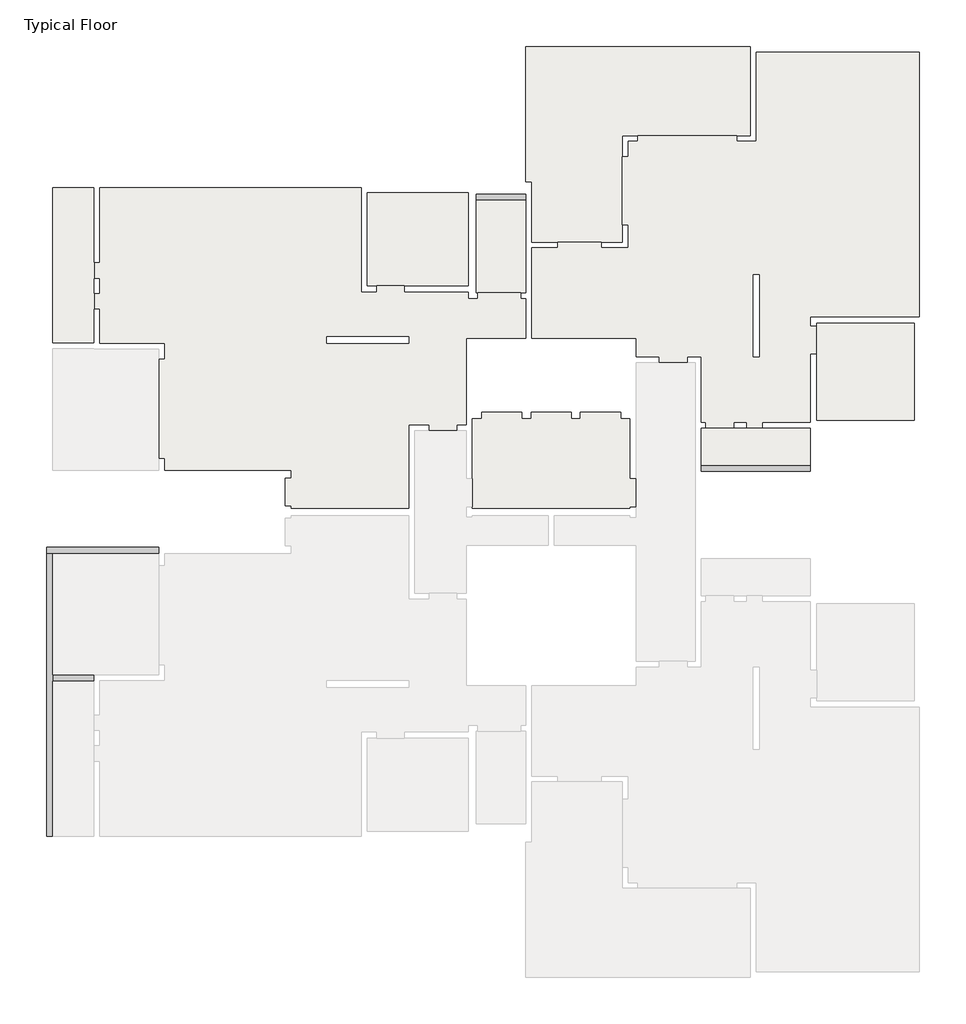
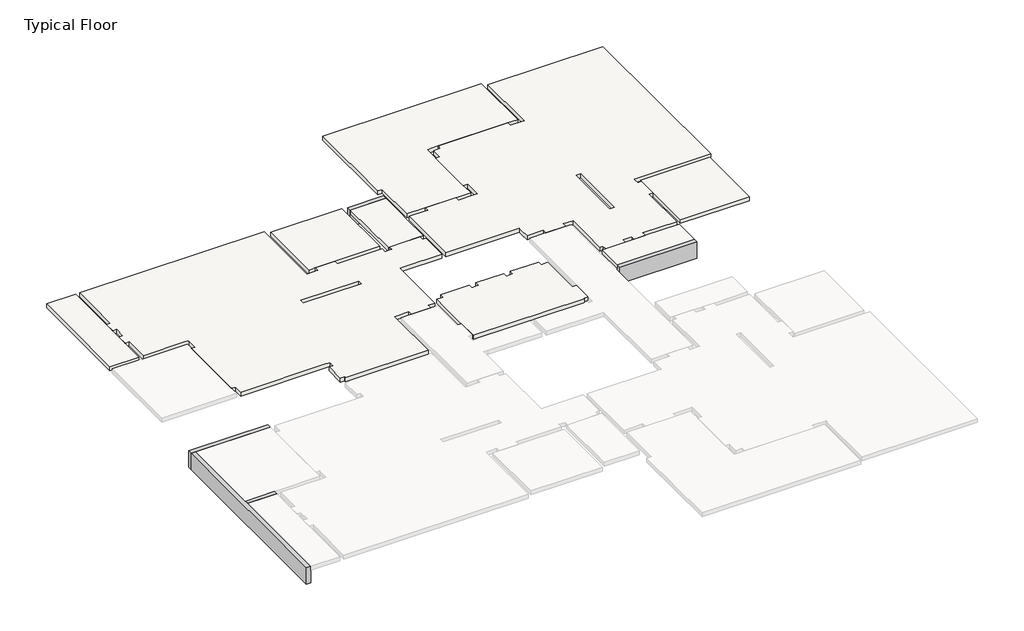
# One storey, part 2 of 2: 9 slabs, 5 beams.
"""IFC4 building model written with IfcOpenShell, lengths in millimetres."""

import ifcopenshell
import ifcopenshell.guid

model = None  # the IFC model being written
_history = None  # IfcOwnerHistory: only IFC2X3 demands one
_inside = {}  # id of a spatial element -> (the spatial element, [elements in it])
_under = {}  # id of a project, library or spatial element -> (it, [spatial elements below it])
_declared = {}  # id of a project -> (the project, [libraries it declares])
_typed = {}  # id of a type object -> (the type object, [elements of that type])
_made_of = {}  # id of a material, layer set ... -> (it, [elements and type objects made of it])


def new_model(schema):
    """Start an empty IFC model of exactly this schema.

    Asked for "IFC4X3", IfcOpenShell would pick the latest addendum, in which some entities
    have other attributes; the version numbers below select the first issue.
    IFC2X3 requires an IfcOwnerHistory on every rooted entity: one is made here for all.
    """
    global model, _history
    if schema == "IFC4X3":
        model = ifcopenshell.file(schema_version=(4, 3, 0, 0))
    else:
        model = ifcopenshell.file(schema=schema)
    _inside.clear()
    _under.clear()
    _declared.clear()
    _typed.clear()
    _made_of.clear()
    _history = None
    if model.schema == "IFC2X3":
        org = make("IfcOrganization", Name="unknown")
        user = make(
            "IfcPersonAndOrganization",
            ThePerson=make("IfcPerson", FamilyName="unknown"),
            TheOrganization=org,
        )
        app = make(
            "IfcApplication",
            ApplicationDeveloper=org,
            Version="unknown",
            ApplicationFullName="unknown",
            ApplicationIdentifier="unknown",
        )
        _history = make(
            "IfcOwnerHistory",
            OwningUser=user,
            OwningApplication=app,
            ChangeAction="ADDED",
            CreationDate=0,
        )
    return model


def make(cls, **values):
    """One entity of the class cls with the attributes given. An attribute that is None is left unset."""
    return model.create_entity(
        cls, **{name: value for name, value in values.items() if value is not None}
    )


def rooted(cls, **values):
    """An entity with a GlobalId (a new one), such as an element, a storey or a relation."""
    return make(cls, GlobalId=ifcopenshell.guid.new(), OwnerHistory=_history, **values)


def si_unit(unit_type, name, prefix=None):
    """IfcSIUnit, for example si_unit("LENGTHUNIT", "METRE", prefix="MILLI")."""
    return make("IfcSIUnit", UnitType=unit_type, Prefix=prefix, Name=name)


def assignment(units):
    """IfcUnitAssignment: the units of a project."""
    return None if units is None else make("IfcUnitAssignment", Units=units)


def point(xyz):
    """IfcCartesianPoint."""
    return None if xyz is None else make("IfcCartesianPoint", Coordinates=xyz)


def direction(xyz):
    """IfcDirection."""
    return None if xyz is None else make("IfcDirection", DirectionRatios=xyz)


def frame(location, z_axis=None, x_axis=None):
    """IfcAxis2Placement3D, a coordinate frame: its origin and axes. An axis left out is left unset."""
    return make(
        "IfcAxis2Placement3D",
        Location=point(location),
        Axis=direction(z_axis),
        RefDirection=direction(x_axis),
    )


def origin():
    """The frame at (0, 0, 0) with its axes left unset."""
    return frame((0.0, 0.0, 0.0))


def place(relative_to, where):
    """IfcLocalPlacement: puts the frame where relative to a parent placement (None: the world)."""
    return make(
        "IfcLocalPlacement", PlacementRelTo=relative_to, RelativePlacement=where
    )


def context(
    kind, dimensions, precision=None, world=None, true_north=None, identifier=None
):
    """IfcGeometricRepresentationContext, for example the 3D "Model" context."""
    return make(
        "IfcGeometricRepresentationContext",
        ContextIdentifier=identifier,
        ContextType=kind,
        CoordinateSpaceDimension=dimensions,
        Precision=precision,
        WorldCoordinateSystem=world,
        TrueNorth=true_north,
    )


def project(units=None, contexts=None):
    """IfcProject with its units and contexts."""
    return rooted(
        "IfcProject",
        Name="project",
        RepresentationContexts=contexts,
        UnitsInContext=assignment(units),
    )


def spatial(cls, under=None, at=None, **own):
    """A site, building, storey or space (cls), placed at a placement, below another one or the project."""
    s = rooted(cls, ObjectPlacement=at, **own)
    if under is not None:
        _under.setdefault(under.id(), (under, []))[1].append(s)
    return s


def faces_of(points, faces, orient=None, outer=None):
    """IfcFace entities. A face is a list of loops; a loop is a list of indices into points, from 0.

    orient and outer hold one flag for each loop. By default every Orientation is true, the
    first loop of a face is its IfcFaceOuterBound and the others are IfcFaceBound.
    """
    made = []
    for i, loops in enumerate(faces):
        bounds = []
        for j, loop in enumerate(loops):
            is_outer = j == 0 if outer is None else outer[i][j]
            bounds.append(
                make(
                    "IfcFaceOuterBound" if is_outer else "IfcFaceBound",
                    Bound=make("IfcPolyLoop", Polygon=[points[k] for k in loop]),
                    Orientation=True if orient is None else orient[i][j],
                )
            )
        made.append(make("IfcFace", Bounds=bounds))
    return made


def faceted_brep(points, faces, orient=None, outer=None, voids=None):
    """IfcFacetedBrep: a solid bounded by flat faces; with voids (closed shells), ...WithVoids."""
    shared = [point(p) for p in points]
    hull = make("IfcClosedShell", CfsFaces=faces_of(shared, faces, orient, outer))
    if voids is None:
        return make("IfcFacetedBrep", Outer=hull)
    return make(
        "IfcFacetedBrepWithVoids",
        Outer=hull,
        Voids=[
            make(cls, CfsFaces=faces_of(shared, fs, o, b)) for cls, fs, o, b in voids
        ],
    )


def shape(context_of_items, identifier, shape_type, items):
    """IfcShapeRepresentation: the items that make up one representation, for example the "Body"."""
    return make(
        "IfcShapeRepresentation",
        ContextOfItems=context_of_items,
        RepresentationIdentifier=identifier,
        RepresentationType=shape_type,
        Items=items,
    )


def made_of(thing, what):
    """Note that an element or type object is made of a material, layer set ...; save() writes the relation."""
    if what is not None:
        _made_of.setdefault(what.id(), (what, []))[1].append(thing)
    return thing


def element(
    cls,
    number,
    at=None,
    inside=None,
    cuts=None,
    type_object=None,
    material=None,
    context=None,
    identifier="Body",
    shape_type=None,
    held_by="IfcProductDefinitionShape",
    body=None,
    shapes=None,
    **own,
):
    """One element of the class cls, such as IfcWall. Its Tag is "e" and its number.

    at: its placement. inside: the storey or other place that contains it. cuts: it is an
    opening in that element (IfcRelVoidsElement). A single representation is given by context,
    identifier, shape_type and body (its items); several are given by shapes. held_by: the class
    of the entity that holds the representations. save() writes the other relations.
    """
    e = rooted(cls, Tag="e%d" % number, ObjectPlacement=at, **own)
    if body is not None:
        shapes = [shape(context, identifier, shape_type, body)]
    if shapes is not None:
        e.Representation = make(held_by, Representations=shapes)
    if inside is not None:
        _inside.setdefault(inside.id(), (inside, []))[1].append(e)
    if cuts is not None:
        rooted(
            "IfcRelVoidsElement", RelatingBuildingElement=cuts, RelatedOpeningElement=e
        )
    if type_object is not None:
        _typed.setdefault(type_object.id(), (type_object, []))[1].append(e)
    return made_of(e, material)


def aggregate(whole, parts):
    """IfcRelAggregates: a whole, such as a stair, and the parts it consists of."""
    return rooted("IfcRelAggregates", RelatingObject=whole, RelatedObjects=parts)


def save(model, path):
    """Write the relations noted so far, then the file.

    IfcRelAggregates (storeys below a building ...), IfcRelContainedInSpatialStructure (elements
    in a storey), IfcRelDefinesByType, IfcRelAssociatesMaterial and IfcRelDeclares: one each for
    every whole, place, type object, material and project.
    """
    for whole, parts in _under.values():
        aggregate(whole, parts)
    for where, things in _inside.values():
        rooted(
            "IfcRelContainedInSpatialStructure",
            RelatedElements=things,
            RelatingStructure=where,
        )
    for kind, things in _typed.values():
        rooted("IfcRelDefinesByType", RelatedObjects=things, RelatingType=kind)
    for what, things in _made_of.values():
        rooted("IfcRelAssociatesMaterial", RelatedObjects=things, RelatingMaterial=what)
    for by, libraries in _declared.values():
        rooted("IfcRelDeclares", RelatingContext=by, RelatedDefinitions=libraries)
    model.write(path)


model = new_model("IFC4")

# Units and contexts
model_context = context("Model", 3, world=origin())
ifc_project = project(units=[si_unit("LENGTHUNIT", "METRE", prefix="MILLI")], contexts=[model_context])

# Site, building, storey
site = spatial("IfcSite", under=ifc_project)
building = spatial("IfcBuilding", under=site)
storey = spatial("IfcBuildingStorey", under=building, Name="Typical Floor", Elevation=3000.0)

# Beams
placement = place(None, origin())
element("IfcBeam", 1, ObjectType="Concrete Rectengular Beam : 20/80", at=placement, inside=storey, context=model_context, shape_type="Brep", body=[
    faceted_brep([(7776.7577342, 13435.0363012, 3000.0), (7776.7577342, 13635.0363012, 3000.0), (4344.3623691, 13635.0363012, 3000.0), (4144.3623691, 13635.0363012, 3000.0), (4144.3623691, 13435.0363012, 3000.0), (4344.3623691, 13435.0363012, 3000.0), (7776.7577342, 13435.0363012, 2200.0), (7776.7577342, 13435.0363012, 2810.0), (4144.3623691, 13435.0363012, 2200.0), (4344.3623691, 13435.0363012, 2200.0), (7776.7577342, 13635.0363012, 2200.0), (4144.3623691, 13635.0363012, 2200.0), (4344.3623691, 13635.0363012, 2200.0)], [[[0, 1, 2, 3, 4, 5]], [[6, 7, 0, 5, 4, 8, 9]], [[10, 6, 9, 8, 11, 12]], [[1, 10, 12, 11, 3, 2]], [[1, 0, 7, 6, 10]], [[4, 3, 11, 8]]]),
])
element("IfcBeam", 2, ObjectType="Concrete Rectengular Beam : 20/80", at=placement, inside=storey, context=model_context, shape_type="Brep", body=[
    faceted_brep([(4144.3623691, 4280.8870961, 3000.0), (4344.3623691, 4280.8870961, 3000.0), (4344.3623691, 9308.461034, 3000.0), (4344.3623691, 9503.461034, 3000.0), (4344.3623691, 13435.0363012, 3000.0), (4144.3623691, 13435.0363012, 3000.0), (4344.3623691, 4280.8870961, 2810.0), (4344.3623691, 4280.8870961, 2200.0), (4344.3623691, 9303.461034, 2200.0), (4344.3623691, 9503.461034, 2200.0), (4344.3623691, 13435.0363012, 2200.0), (4344.3623691, 13435.0363012, 2810.0), (4144.3623691, 4280.8870961, 2200.0), (4144.3623691, 13435.0363012, 2200.0)], [[[0, 1, 2, 3, 4, 5]], [[1, 6, 7, 8, 9, 10, 11, 4, 3, 2]], [[7, 12, 13, 10, 9, 8]], [[12, 0, 5, 13]], [[1, 0, 12, 7, 6]], [[5, 4, 11, 10, 13]]]),
])
element("IfcBeam", 3, ObjectType="Concrete Rectengular Beam : 20/80", at=placement, inside=storey, context=model_context, shape_type="Brep", body=[
    faceted_brep([(5676.0285364, 9503.461034, 3000.0), (4344.3623691, 9503.461034, 3000.0), (4344.3623691, 9308.461034, 3000.0), (5676.0285364, 9308.461034, 3000.0), (4344.3623691, 9303.461034, 2200.0), (5676.0285364, 9303.461034, 2200.0), (5676.0285364, 9303.461034, 2810.0), (4344.3623691, 9303.461034, 2810.0), (5676.0285364, 9503.461034, 2200.0), (4344.3623691, 9503.461034, 2200.0), (4344.3623691, 9503.461034, 2810.0), (5676.0285364, 9308.461034, 2810.0), (4344.3623691, 9308.461034, 2810.0)], [[[0, 1, 2, 3]], [[4, 5, 6, 7]], [[8, 5, 4, 9]], [[9, 10, 1, 0, 8]], [[5, 8, 0, 3, 11, 6]], [[9, 4, 7, 12, 2, 1, 10]], [[11, 12, 7, 6]], [[12, 11, 3, 2]]]),
])
element("IfcBeam", 4, ObjectType="Concrete Rectengular Beam : 20/80", at=placement, inside=storey, context=model_context, shape_type="Brep", body=[
    faceted_brep([(28875.6979001, 16096.9481981, 3000.0), (28875.6979001, 16296.9481981, 3000.0), (25344.8278571, 16296.9481981, 3000.0), (25344.8278571, 16096.9481981, 3000.0), (28875.6979001, 16096.9481981, 2200.0), (25344.8278571, 16096.9481981, 2200.0), (28875.6979001, 16296.9481981, 2200.0), (25344.8278571, 16296.9481981, 2200.0), (28875.6979001, 16296.9481981, 2810.0), (25344.8278571, 16296.9481981, 2810.0)], [[[0, 1, 2, 3]], [[4, 0, 3, 5]], [[6, 4, 5, 7]], [[1, 8, 6, 7, 9, 2]], [[1, 0, 4, 6, 8]], [[3, 2, 9, 7, 5]]]),
])
element("IfcBeam", 5, ObjectType="Concrete Rectengular Beam : 20/80", at=placement, inside=storey, context=model_context, shape_type="Brep", body=[
    faceted_brep([(19662.6522503, 24869.2786346, 3000.0), (19662.6522503, 25069.2786346, 3000.0), (18051.1049523, 25069.2786346, 3000.0), (18051.1049523, 24869.2786346, 3000.0), (19662.6522503, 25069.2786346, 2200.0), (18051.1049523, 25069.2786346, 2200.0), (19662.6522503, 24869.2786346, 2200.0), (18051.1049523, 24869.2786346, 2200.0), (19662.6522503, 24869.2786346, 2810.0), (18051.1049523, 24869.2786346, 2810.0)], [[[0, 1, 2, 3]], [[1, 4, 5, 2]], [[4, 6, 7, 5]], [[6, 8, 0, 3, 9, 7]], [[1, 0, 8, 6, 4]], [[3, 2, 5, 7, 9]]]),
])

# Slabs
element("IfcSlab", 6, ObjectType="19", at=placement, inside=storey, context=model_context, shape_type="Brep", body=[
    faceted_brep([(4344.3623691, 20253.0459905, 2810.0), (4344.3623691, 20258.0459905, 2810.0), (4344.3623691, 25280.6199284, 2810.0), (5676.0285364, 25280.6199284, 2810.0), (5676.0285364, 22851.8697843, 2810.0), (5681.0285364, 22851.8697843, 2810.0), (5681.0285364, 22352.6390151, 2810.0), (5676.0285364, 22352.6390151, 2810.0), (5676.0285364, 21853.4082459, 2810.0), (5681.0285364, 21853.4082459, 2810.0), (5681.0285364, 21354.1774766, 2810.0), (5676.0285364, 21354.1774766, 2810.0), (5676.0285364, 20258.0459905, 2810.0), (5676.0285364, 20253.0459905, 2810.0), (4344.3623691, 25280.6199284, 3000.0), (4344.3623691, 20253.0459905, 3000.0), (5676.0285364, 20253.0459905, 3000.0), (5676.0285364, 21354.1774766, 3000.0), (5681.0285364, 21354.1774766, 3000.0), (5681.0285364, 21853.4082459, 3000.0), (5676.0285364, 21853.4082459, 3000.0), (5676.0285364, 22352.6390151, 3000.0), (5681.0285364, 22352.6390151, 3000.0), (5681.0285364, 22851.8697843, 3000.0), (5676.0285364, 22851.8697843, 3000.0), (5676.0285364, 25280.6199284, 3000.0)], [[[0, 1, 2, 3, 4, 5, 6, 7, 8, 9, 10, 11, 12, 13]], [[14, 15, 16, 17, 18, 19, 20, 21, 22, 23, 24, 25]], [[18, 10, 9, 19]], [[5, 23, 22, 6]], [[15, 0, 13, 16]], [[2, 1, 0, 15, 14]], [[2, 14, 25, 3]], [[11, 17, 16, 13, 12]], [[17, 11, 10, 18]], [[24, 4, 3, 25]], [[4, 24, 23, 5]], [[7, 21, 20, 8]], [[8, 20, 19, 9]], [[21, 7, 6, 22]]]),
])
element("IfcSlab", 7, ObjectType="19", at=placement, inside=storey, context=model_context, shape_type="Brep", body=[
    faceted_brep([(5866.0285364, 22851.8697843, 2810.0), (5866.0285364, 25280.6199284, 2810.0), (14329.4188071, 25280.6199284, 2810.0), (14329.4188071, 22100.4193798, 2810.0), (14329.4188071, 21900.4193798, 2810.0), (14830.1280269, 21900.4193798, 2810.0), (14830.1280269, 22100.4193798, 2810.0), (15730.1380159, 22100.4193798, 2810.0), (15730.1380159, 21900.4193798, 2810.0), (17801.1049523, 21900.4193798, 2810.0), (17801.1049523, 21878.6523235, 2810.0), (17801.1049523, 21688.6523235, 2810.0), (18101.9290458, 21688.6523235, 2810.0), (18101.9290458, 21878.6523235, 2810.0), (19501.7092875, 21878.6523235, 2810.0), (19501.7092875, 21688.6523235, 2810.0), (19662.6522503, 21688.6523235, 2810.0), (19662.6522503, 20409.5793039, 2810.0), (17931.3366974, 20409.5793039, 2810.0), (17731.3366974, 20409.5793039, 2810.0), (17731.3366974, 17607.9011498, 2810.0), (17430.6274775, 17607.9011498, 2810.0), (17430.6274775, 17407.9011498, 2810.0), (16530.6174885, 17407.9011498, 2810.0), (16530.6174885, 17607.9011498, 2810.0), (15871.0829765, 17607.9011498, 2810.0), (15871.0829765, 17407.9011498, 2810.0), (15871.0829765, 14905.7535122, 2810.0), (12068.6856136, 14905.7535122, 2810.0), (12068.6856136, 14975.6366408, 2810.0), (11878.6856136, 14975.6366408, 2810.0), (11878.6856136, 15877.7643004, 2810.0), (12068.6856136, 15877.7643004, 2810.0), (12068.6856136, 16126.4707233, 2810.0), (11878.6856136, 16126.4707233, 2810.0), (7966.7577342, 16126.4707233, 2810.0), (7966.7577342, 16527.889163, 2810.0), (7776.7577342, 16527.889163, 2810.0), (7776.7577342, 19727.6893828, 2810.0), (7966.7577342, 19727.6893828, 2810.0), (7966.7577342, 20248.0459905, 2810.0), (7776.7577342, 20248.0459905, 2810.0), (5866.0285364, 20248.0459905, 2810.0), (5866.0285364, 21354.1774766, 2810.0), (5681.0285364, 21354.1774766, 2810.0), (5681.0285364, 21853.4082459, 2810.0), (5866.0285364, 21853.4082459, 2810.0), (5866.0285364, 22352.6390151, 2810.0), (5681.0285364, 22352.6390151, 2810.0), (5681.0285364, 22851.8697843, 2810.0), (15869.904273, 20448.6363411, 2810.0), (13218.5807289, 20448.6363411, 2810.0), (13218.5807289, 20248.6363411, 2810.0), (15869.904273, 20248.6363411, 2810.0), (5866.0285364, 25280.6199284, 3000.0), (5866.0285364, 22851.8697843, 3000.0), (5681.0285364, 22851.8697843, 3000.0), (5681.0285364, 22352.6390151, 3000.0), (5866.0285364, 22352.6390151, 3000.0), (5866.0285364, 21853.4082459, 3000.0), (5681.0285364, 21853.4082459, 3000.0), (5681.0285364, 21354.1774766, 3000.0), (5866.0285364, 21354.1774766, 3000.0), (5866.0285364, 20248.0459905, 3000.0), (7776.7577342, 20248.0459905, 3000.0), (7966.7577342, 20248.0459905, 3000.0), (7966.7577342, 19727.6893828, 3000.0), (7776.7577342, 19727.6893828, 3000.0), (7776.7577342, 16527.889163, 3000.0), (7966.7577342, 16527.889163, 3000.0), (7966.7577342, 16126.4707233, 3000.0), (11878.6856136, 16126.4707233, 3000.0), (12068.6856136, 16126.4707233, 3000.0), (12068.6856136, 15877.7643004, 3000.0), (11878.6856136, 15877.7643004, 3000.0), (11878.6856136, 14975.6366408, 3000.0), (12068.6856136, 14975.6366408, 3000.0), (12068.6856136, 14905.7535122, 3000.0), (15871.0829765, 14905.7535122, 3000.0), (15871.0829765, 17407.9011498, 3000.0), (15871.0829765, 17607.9011498, 3000.0), (16530.6174885, 17607.9011498, 3000.0), (16530.6174885, 17407.9011498, 3000.0), (17430.6274775, 17407.9011498, 3000.0), (17430.6274775, 17607.9011498, 3000.0), (17731.3366974, 17607.9011498, 3000.0), (17731.3366974, 20409.5793039, 3000.0), (17931.3366974, 20409.5793039, 3000.0), (19662.6522503, 20409.5793039, 3000.0), (19662.6522503, 21688.6523235, 3000.0), (19501.7092875, 21688.6523235, 3000.0), (19501.7092875, 21878.6523235, 3000.0), (18101.9290458, 21878.6523235, 3000.0), (18101.9290458, 21688.6523235, 3000.0), (17801.1049523, 21688.6523235, 3000.0), (17801.1049523, 21878.6523235, 3000.0), (17801.1049523, 21900.4193798, 3000.0), (15730.1380159, 21900.4193798, 3000.0), (15730.1380159, 22100.4193798, 3000.0), (14830.1280269, 22100.4193798, 3000.0), (14830.1280269, 21900.4193798, 3000.0), (14329.4188071, 21900.4193798, 3000.0), (14329.4188071, 22100.4193798, 3000.0), (14329.4188071, 25280.6199284, 3000.0), (13218.5807289, 20448.6363411, 3000.0), (15869.904273, 20448.6363411, 3000.0), (15869.904273, 20248.6363411, 3000.0), (13218.5807289, 20248.6363411, 3000.0)], [[[0, 1, 2, 3, 4, 5, 6, 7, 8, 9, 10, 11, 12, 13, 14, 15, 16, 17, 18, 19, 20, 21, 22, 23, 24, 25, 26, 27, 28, 29, 30, 31, 32, 33, 34, 35, 36, 37, 38, 39, 40, 41, 42, 43, 44, 45, 46, 47, 48, 49], [50, 51, 52, 53]], [[54, 55, 56, 57, 58, 59, 60, 61, 62, 63, 64, 65, 66, 67, 68, 69, 70, 71, 72, 73, 74, 75, 76, 77, 78, 79, 80, 81, 82, 83, 84, 85, 86, 87, 88, 89, 90, 91, 92, 93, 94, 95, 96, 97, 98, 99, 100, 101, 102, 103], [104, 105, 106, 107]], [[1, 0, 55, 54]], [[2, 1, 54, 103]], [[2, 103, 102, 101, 4, 3]], [[5, 4, 101, 100]], [[6, 5, 100, 99]], [[7, 6, 99, 98]], [[8, 7, 98, 97]], [[9, 8, 97, 96]], [[9, 96, 95, 94, 11, 10]], [[12, 11, 94, 93]], [[13, 12, 93, 92]], [[14, 13, 92, 91]], [[15, 14, 91, 90]], [[16, 15, 90, 89]], [[17, 16, 89, 88]], [[17, 88, 87, 86, 19, 18]], [[20, 19, 86, 85]], [[21, 20, 85, 84]], [[22, 21, 84, 83]], [[23, 22, 83, 82]], [[24, 23, 82, 81]], [[25, 24, 81, 80]], [[25, 80, 79, 78, 27, 26]], [[28, 27, 78, 77]], [[29, 28, 77, 76]], [[30, 29, 76, 75]], [[31, 30, 75, 74]], [[32, 31, 74, 73]], [[33, 32, 73, 72]], [[33, 72, 71, 70, 35, 34]], [[36, 35, 70, 69]], [[37, 36, 69, 68]], [[38, 37, 68, 67]], [[39, 38, 67, 66]], [[40, 39, 66, 65]], [[40, 65, 64, 63, 42, 41]], [[43, 42, 63, 62]], [[43, 62, 61, 44]], [[59, 46, 45, 60]], [[47, 46, 59, 58]], [[47, 58, 57, 48]], [[55, 0, 49, 56]], [[51, 50, 105, 104]], [[52, 51, 104, 107]], [[53, 52, 107, 106]], [[50, 53, 106, 105]], [[45, 44, 61, 60]], [[49, 48, 57, 56]]]),
])
element("IfcSlab", 8, ObjectType="19", at=placement, inside=storey, context=model_context, shape_type="Brep", body=[
    faceted_brep([(23233.0448184, 20409.5793039, 2810.0), (19852.6522503, 20409.5793039, 2810.0), (19852.6522503, 23329.8470094, 2810.0), (20702.4284964, 23329.8470094, 2810.0), (20702.4284964, 23519.8470094, 2810.0), (22104.3264087, 23519.8470094, 2810.0), (22104.3264087, 23329.8470094, 2810.0), (22784.6890098, 23329.8470094, 2810.0), (22974.6890098, 23329.8470094, 2810.0), (22974.6890098, 24081.620059, 2810.0), (22784.6890098, 24081.620059, 2810.0), (22784.0986592, 24081.620059, 2810.0), (22784.0986592, 26281.8797734, 2810.0), (22974.0986592, 26281.8797734, 2810.0), (22974.0986592, 26781.6500261, 2810.0), (23288.1042531, 26781.6500261, 2810.0), (23288.1042531, 26971.6500261, 2810.0), (26490.0221434, 26971.6500261, 2810.0), (26490.0221434, 26781.6500261, 2810.0), (27124.7329615, 26781.6500261, 2810.0), (27124.7329615, 26971.6500261, 2810.0), (27124.7329615, 29662.2723415, 2810.0), (32407.3840453, 29662.2723415, 2810.0), (32407.3840453, 21099.9399072, 2810.0), (29076.6368672, 21099.9399072, 2810.0), (28876.6368672, 21099.9399072, 2810.0), (28876.6368672, 20799.2306873, 2810.0), (29076.6368672, 20799.2306873, 2810.0), (29076.6368672, 19899.2206983, 2810.0), (28876.6368672, 19899.2206983, 2810.0), (28876.6368672, 17688.3726312, 2810.0), (27326.5020155, 17688.3726312, 2810.0), (27326.5020155, 17488.3726312, 2810.0), (26824.6140922, 17488.3726312, 2810.0), (26824.6140922, 17688.3726312, 2810.0), (26394.7269681, 17688.3726312, 2810.0), (26394.7269681, 17488.3726312, 2810.0), (25494.7169791, 17488.3726312, 2810.0), (25494.7169791, 17688.3726312, 2810.0), (25344.8278571, 17688.3726312, 2810.0), (25344.8278571, 19609.0998313, 2810.0), (25344.8278571, 19809.0998313, 2810.0), (24884.8278571, 19809.0998313, 2810.0), (24884.8278571, 19609.0998313, 2810.0), (23984.8178681, 19609.0998313, 2810.0), (23984.8178681, 19809.0998313, 2810.0), (23233.0448184, 19809.0998313, 2810.0), (23233.0448184, 20209.5793039, 2810.0), (27225.7927957, 19808.1608642, 2810.0), (27225.7927957, 22459.4844083, 2810.0), (27025.7927957, 22459.4844083, 2810.0), (27025.7927957, 19808.1608642, 2810.0), (19852.6522503, 20409.5793039, 3000.0), (23233.0448184, 20409.5793039, 3000.0), (23233.0448184, 20209.5793039, 3000.0), (23233.0448184, 19809.0998313, 3000.0), (23984.8178681, 19809.0998313, 3000.0), (23984.8178681, 19609.0998313, 3000.0), (24884.8278571, 19609.0998313, 3000.0), (24884.8278571, 19809.0998313, 3000.0), (25344.8278571, 19809.0998313, 3000.0), (25344.8278571, 19609.0998313, 3000.0), (25344.8278571, 17688.3726312, 3000.0), (25494.7169791, 17688.3726312, 3000.0), (25494.7169791, 17488.3726312, 3000.0), (26394.7269681, 17488.3726312, 3000.0), (26394.7269681, 17688.3726312, 3000.0), (26824.6140922, 17688.3726312, 3000.0), (26824.6140922, 17488.3726312, 3000.0), (27326.5020155, 17488.3726312, 3000.0), (27326.5020155, 17688.3726312, 3000.0), (28876.6368672, 17688.3726312, 3000.0), (28876.6368672, 19899.2206983, 3000.0), (29076.6368672, 19899.2206983, 3000.0), (29076.6368672, 20799.2306873, 3000.0), (28876.6368672, 20799.2306873, 3000.0), (28876.6368672, 21099.9399072, 3000.0), (29076.6368672, 21099.9399072, 3000.0), (32407.3840453, 21099.9399072, 3000.0), (32407.3840453, 29662.2723415, 3000.0), (27124.7329615, 29662.2723415, 3000.0), (27124.7329615, 26971.6500261, 3000.0), (27124.7329615, 26781.6500261, 3000.0), (26490.0221434, 26781.6500261, 3000.0), (26490.0221434, 26971.6500261, 3000.0), (23288.1042531, 26971.6500261, 3000.0), (23288.1042531, 26781.6500261, 3000.0), (22974.0986592, 26781.6500261, 3000.0), (22974.0986592, 26281.8797734, 3000.0), (22784.0986592, 26281.8797734, 3000.0), (22784.0986592, 24081.620059, 3000.0), (22784.6890098, 24081.620059, 3000.0), (22974.6890098, 24081.620059, 3000.0), (22974.6890098, 23329.8470094, 3000.0), (22784.6890098, 23329.8470094, 3000.0), (22104.3264087, 23329.8470094, 3000.0), (22104.3264087, 23519.8470094, 3000.0), (20702.4284964, 23519.8470094, 3000.0), (20702.4284964, 23329.8470094, 3000.0), (19852.6522503, 23329.8470094, 3000.0), (27225.7927957, 22459.4844083, 3000.0), (27225.7927957, 19808.1608642, 3000.0), (27025.7927957, 19808.1608642, 3000.0), (27025.7927957, 22459.4844083, 3000.0)], [[[0, 1, 2, 3, 4, 5, 6, 7, 8, 9, 10, 11, 12, 13, 14, 15, 16, 17, 18, 19, 20, 21, 22, 23, 24, 25, 26, 27, 28, 29, 30, 31, 32, 33, 34, 35, 36, 37, 38, 39, 40, 41, 42, 43, 44, 45, 46, 47], [48, 49, 50, 51]], [[52, 53, 54, 55, 56, 57, 58, 59, 60, 61, 62, 63, 64, 65, 66, 67, 68, 69, 70, 71, 72, 73, 74, 75, 76, 77, 78, 79, 80, 81, 82, 83, 84, 85, 86, 87, 88, 89, 90, 91, 92, 93, 94, 95, 96, 97, 98, 99], [100, 101, 102, 103]], [[1, 0, 53, 52]], [[2, 1, 52, 99]], [[3, 2, 99, 98]], [[4, 3, 98, 97]], [[5, 4, 97, 96]], [[6, 5, 96, 95]], [[6, 95, 94, 93, 8, 7]], [[9, 8, 93, 92]], [[9, 92, 91, 90, 11, 10]], [[12, 11, 90, 89]], [[13, 12, 89, 88]], [[14, 13, 88, 87]], [[15, 14, 87, 86]], [[16, 15, 86, 85]], [[17, 16, 85, 84]], [[18, 17, 84, 83]], [[19, 18, 83, 82]], [[19, 82, 81, 80, 21, 20]], [[22, 21, 80, 79]], [[23, 22, 79, 78]], [[23, 78, 77, 76, 25, 24]], [[26, 25, 76, 75]], [[27, 26, 75, 74]], [[28, 27, 74, 73]], [[29, 28, 73, 72]], [[30, 29, 72, 71]], [[31, 30, 71, 70]], [[32, 31, 70, 69]], [[33, 32, 69, 68]], [[34, 33, 68, 67]], [[35, 34, 67, 66]], [[36, 35, 66, 65]], [[37, 36, 65, 64]], [[38, 37, 64, 63]], [[39, 38, 63, 62]], [[39, 62, 61, 60, 41, 40]], [[42, 41, 60, 59]], [[43, 42, 59, 58]], [[44, 43, 58, 57]], [[45, 44, 57, 56]], [[46, 45, 56, 55]], [[46, 55, 54, 53, 0, 47]], [[48, 101, 100, 49]], [[50, 103, 102, 51]], [[49, 100, 103, 50]], [[101, 48, 51, 102]]]),
])
element("IfcSlab", 9, ObjectType="19", at=placement, inside=storey, context=model_context, shape_type="Brep", body=[
    faceted_brep([(29076.6368672, 20899.9399072, 2810.0), (32247.3840453, 20899.9399072, 2810.0), (32247.3840453, 17747.7822806, 2810.0), (29076.6368672, 17747.7822806, 2810.0), (29076.6368672, 19899.2206983, 2810.0), (29076.6368672, 20799.2306873, 2810.0), (32247.3840453, 20899.9399072, 3000.0), (29076.6368672, 20899.9399072, 3000.0), (29076.6368672, 20799.2306873, 3000.0), (29076.6368672, 19899.2206983, 3000.0), (29076.6368672, 17747.7822806, 3000.0), (32247.3840453, 17747.7822806, 3000.0)], [[[0, 1, 2, 3, 4, 5]], [[6, 7, 8, 9, 10, 11]], [[1, 0, 7, 6]], [[2, 1, 6, 11]], [[3, 2, 11, 10]], [[3, 10, 9, 8, 7, 0, 5, 4]]]),
])
element("IfcSlab", 10, ObjectType="19", at=placement, inside=storey, context=model_context, shape_type="Brep", body=[
    faceted_brep([(19662.6522503, 29852.2723415, 2810.0), (26934.7329615, 29852.2723415, 2810.0), (26934.7329615, 26971.6500261, 2810.0), (26490.0221434, 26971.6500261, 2810.0), (23288.1042531, 26971.6500261, 2810.0), (22784.0986592, 26971.6500261, 2810.0), (22784.0986592, 26281.8797734, 2810.0), (22784.0986592, 24081.620059, 2810.0), (22784.6890098, 24081.620059, 2810.0), (22784.6890098, 23519.8470094, 2810.0), (22104.3264087, 23519.8470094, 2810.0), (20702.4284964, 23519.8470094, 2810.0), (19852.6522503, 23519.8470094, 2810.0), (19852.6522503, 25470.811948, 2810.0), (19662.6522503, 25470.811948, 2810.0), (26934.7329615, 29852.2723415, 3000.0), (19662.6522503, 29852.2723415, 3000.0), (19662.6522503, 25470.811948, 3000.0), (19852.6522503, 25470.811948, 3000.0), (19852.6522503, 23519.8470094, 3000.0), (20702.4284964, 23519.8470094, 3000.0), (22104.3264087, 23519.8470094, 3000.0), (22784.6890098, 23519.8470094, 3000.0), (22784.6890098, 24081.620059, 3000.0), (22784.0986592, 24081.620059, 3000.0), (22784.0986592, 26281.8797734, 3000.0), (22784.0986592, 26971.6500261, 3000.0), (22974.0986592, 26971.6500261, 3000.0), (23288.1042531, 26971.6500261, 3000.0), (26490.0221434, 26971.6500261, 3000.0), (26934.7329615, 26971.6500261, 3000.0), (26934.7329615, 29662.2723415, 3000.0)], [[[0, 1, 2, 3, 4, 5, 6, 7, 8, 9, 10, 11, 12, 13, 14]], [[15, 16, 17, 18, 19, 20, 21, 22, 23, 24, 25, 26, 27, 28, 29, 30, 31]], [[1, 0, 16, 15]], [[2, 1, 15, 31, 30]], [[2, 30, 29, 28, 27, 26, 5, 4, 3]], [[19, 12, 11, 10, 9, 22, 21, 20]], [[13, 12, 19, 18]], [[14, 13, 18, 17]], [[0, 14, 17, 16]], [[5, 26, 25, 24, 7, 6]], [[9, 8, 23, 22]], [[7, 24, 23, 8]]]),
])
element("IfcSlab", 11, ObjectType="19", at=placement, inside=storey, context=model_context, shape_type="Brep", body=[
    faceted_brep([(14529.4188071, 22100.4193798, 2810.0), (14529.4188071, 25120.7159382, 2810.0), (17801.1049523, 25120.7159382, 2810.0), (17801.1049523, 22100.4193798, 2810.0), (15730.1380159, 22100.4193798, 2810.0), (14830.1280269, 22100.4193798, 2810.0), (14529.4188071, 25120.7159382, 3000.0), (14529.4188071, 22100.4193798, 3000.0), (14830.1280269, 22100.4193798, 3000.0), (15730.1380159, 22100.4193798, 3000.0), (17801.1049523, 22100.4193798, 3000.0), (17801.1049523, 25120.7159382, 3000.0)], [[[0, 1, 2, 3, 4, 5]], [[6, 7, 8, 9, 10, 11]], [[7, 0, 5, 4, 3, 10, 9, 8]], [[1, 0, 7, 6]], [[2, 1, 6, 11]], [[3, 2, 11, 10]]]),
])
element("IfcSlab", 12, ObjectType="19", at=placement, inside=storey, context=model_context, shape_type="Brep", body=[
    faceted_brep([(17931.3366974, 17808.1408861, 2810.0), (18231.1069501, 17808.1408861, 2810.0), (18231.1069501, 18008.1408861, 2810.0), (19531.3566754, 18008.1408861, 2810.0), (19531.3566754, 17808.1408861, 2810.0), (19832.0658953, 17808.1408861, 2810.0), (19832.0658953, 18008.1408861, 2810.0), (21132.3156206, 18008.1408861, 2810.0), (21132.3156206, 17808.1408861, 2810.0), (21433.0248404, 17808.1408861, 2810.0), (21433.0248404, 18008.1408861, 2810.0), (22733.2745657, 18008.1408861, 2810.0), (22733.2745657, 17808.1408861, 2810.0), (23033.0448184, 17808.1408861, 2810.0), (23033.0448184, 15856.5875947, 2810.0), (23233.0448184, 15856.5875947, 2810.0), (23233.0448184, 14956.5776057, 2810.0), (23033.0448184, 14956.5776057, 2810.0), (23033.0448184, 14905.8683859, 2810.0), (17931.3366974, 14905.8683859, 2810.0), (17931.3366974, 14956.5776057, 2810.0), (17931.3366974, 15852.9011498, 2810.0), (18231.1069501, 17808.1408861, 3000.0), (17931.3366974, 17808.1408861, 3000.0), (17931.3366974, 15852.9011498, 3000.0), (17931.3366974, 14956.5776057, 3000.0), (17931.3366974, 14905.8683859, 3000.0), (23033.0448184, 14905.8683859, 3000.0), (23033.0448184, 14956.5776057, 3000.0), (23233.0448184, 14956.5776057, 3000.0), (23233.0448184, 15856.5875947, 3000.0), (23033.0448184, 15856.5875947, 3000.0), (23033.0448184, 17808.1408861, 3000.0), (22733.2745657, 17808.1408861, 3000.0), (22733.2745657, 18008.1408861, 3000.0), (21433.0248404, 18008.1408861, 3000.0), (21433.0248404, 17808.1408861, 3000.0), (21132.3156206, 17808.1408861, 3000.0), (21132.3156206, 18008.1408861, 3000.0), (19832.0658953, 18008.1408861, 3000.0), (19832.0658953, 17808.1408861, 3000.0), (19531.3566754, 17808.1408861, 3000.0), (19531.3566754, 18008.1408861, 3000.0), (18231.1069501, 18008.1408861, 3000.0)], [[[0, 1, 2, 3, 4, 5, 6, 7, 8, 9, 10, 11, 12, 13, 14, 15, 16, 17, 18, 19, 20, 21]], [[22, 23, 24, 25, 26, 27, 28, 29, 30, 31, 32, 33, 34, 35, 36, 37, 38, 39, 40, 41, 42, 43]], [[1, 0, 23, 22]], [[2, 1, 22, 43]], [[3, 2, 43, 42]], [[4, 3, 42, 41]], [[5, 4, 41, 40]], [[6, 5, 40, 39]], [[7, 6, 39, 38]], [[8, 7, 38, 37]], [[9, 8, 37, 36]], [[10, 9, 36, 35]], [[11, 10, 35, 34]], [[12, 11, 34, 33]], [[13, 12, 33, 32]], [[14, 13, 32, 31]], [[15, 14, 31, 30]], [[16, 15, 30, 29]], [[17, 16, 29, 28]], [[18, 17, 28, 27]], [[19, 18, 27, 26]], [[19, 26, 25, 24, 23, 0, 21, 20]]]),
])
element("IfcSlab", 13, ObjectType="19", at=placement, inside=storey, context=model_context, shape_type="Brep", body=[
    faceted_brep([(19662.6522503, 24869.2786346, 2810.0), (19662.6522503, 21878.6523235, 2810.0), (19501.7092875, 21878.6523235, 2810.0), (18101.9290458, 21878.6523235, 2810.0), (18051.1049523, 21878.6523235, 2810.0), (18051.1049523, 24869.2786346, 2810.0), (19662.6522503, 21878.6523235, 3000.0), (19662.6522503, 23329.8470094, 3000.0), (19662.6522503, 23519.8470094, 3000.0), (19662.6522503, 24869.2786346, 3000.0), (18051.1049523, 24869.2786346, 3000.0), (18051.1049523, 21878.6523235, 3000.0), (18101.9290458, 21878.6523235, 3000.0), (19501.7092875, 21878.6523235, 3000.0)], [[[0, 1, 2, 3, 4, 5]], [[6, 7, 8, 9, 10, 11, 12, 13]], [[1, 0, 9, 8, 7, 6]], [[0, 5, 10, 9]], [[5, 4, 11, 10]], [[11, 4, 3, 2, 1, 6, 13, 12]]]),
])
element("IfcSlab", 14, ObjectType="19", at=placement, inside=storey, context=model_context, shape_type="Brep", body=[
    faceted_brep([(28875.6979001, 16296.9481981, 2810.0), (25344.8278571, 16296.9481981, 2810.0), (25344.8278571, 17488.3726312, 2810.0), (25494.7169791, 17488.3726312, 2810.0), (26394.7269681, 17488.3726312, 2810.0), (26824.6140922, 17488.3726312, 2810.0), (27326.5020155, 17488.3726312, 2810.0), (28875.6979001, 17488.3726312, 2810.0), (28875.6979001, 16296.9481981, 3000.0), (28875.6979001, 17488.3726312, 3000.0), (27326.5020155, 17488.3726312, 3000.0), (26824.6140922, 17488.3726312, 3000.0), (26394.7269681, 17488.3726312, 3000.0), (25494.7169791, 17488.3726312, 3000.0), (25344.8278571, 17488.3726312, 3000.0), (25344.8278571, 16296.9481981, 3000.0)], [[[0, 1, 2, 3, 4, 5, 6, 7]], [[8, 9, 10, 11, 12, 13, 14, 15]], [[0, 7, 9, 8]], [[7, 6, 5, 4, 3, 2, 14, 13, 12, 11, 10, 9]], [[2, 1, 15, 14]], [[1, 0, 8, 15]]]),
])

save(model, "model.ifc")

# Revit data of these elements
# Type "Concrete Rectengular Beam : 20/80"
#   Length [instance default] = 152.4 cm
#   b = 20 cm
#   h = 80 cm
#   Structural Material [instance default] = Concrete
#   Assembly Code = ""
# Type "19"
#   Function = 0
#   Layers, outside or top first: 19 cm "Concrete" (function 1)
# Element 1 (IfcBeam, "Concrete Rectengular Beam : 20/80")
#   Comments = ""
#   Mark = "B4"
#   SOFiSTiK_AMG_Comments = ""
#   SOFiSTiK_AMG_Scheduled = yes
#   SOFiSTiK_AMG_Adjusted = yes
#   Structural Material = Concrete
#   Phase Created = New Construction
#   Materials on its faces: "Concrete"
# Element 2 (IfcBeam, "Concrete Rectengular Beam : 20/80")
#   Comments = ""
#   Mark = "B5"
#   SOFiSTiK_AMG_Comments = ""
#   SOFiSTiK_AMG_Scheduled = yes
#   SOFiSTiK_AMG_Adjusted = yes
#   Structural Material = Concrete
#   Phase Created = New Construction
#   Materials on its faces: "Concrete"
# Element 3 (IfcBeam, "Concrete Rectengular Beam : 20/80")
#   Comments = ""
#   Mark = "B6"
#   SOFiSTiK_AMG_Comments = ""
#   SOFiSTiK_AMG_Scheduled = yes
#   SOFiSTiK_AMG_Adjusted = yes
#   Structural Material = Concrete
#   Phase Created = New Construction
#   Materials on its faces: "Concrete"
# Element 4 (IfcBeam, "Concrete Rectengular Beam : 20/80")
#   Comments = ""
#   Mark = "B10"
#   SOFiSTiK_AMG_Comments = ""
#   SOFiSTiK_AMG_Scheduled = yes
#   SOFiSTiK_AMG_Adjusted = yes
#   Structural Material = Concrete
#   Phase Created = New Construction
#   Materials on its faces: "Concrete"
# Element 5 (IfcBeam, "Concrete Rectengular Beam : 20/80")
#   Comments = ""
#   Mark = "B11"
#   SOFiSTiK_AMG_Comments = ""
#   SOFiSTiK_AMG_Scheduled = yes
#   SOFiSTiK_AMG_Adjusted = yes
#   Structural Material = Concrete
#   Phase Created = New Construction
#   Materials on its faces: "Concrete"
# Element 6 (IfcSlab, "19")
#   Mark = "S2"
#   SOFiSTiK_AMG_Comments = ""
#   Height Offset From Level = 0 cm
#   built-in parameter 1001954 = 1
#   SOFiSTiK_AMG_Scheduled = yes
#   SOFiSTiK_AMG_Adjusted = yes
#   Phase Created = New Construction
#   Materials on its faces: "Concrete"
# Element 7 (IfcSlab, "19")
#   Mark = "S3"
#   SOFiSTiK_AMG_Comments = ""
#   built-in parameter 1001955 = -1.5708 (stored number, unit not read)
#   Height Offset From Level = 0 cm
#   built-in parameter 1001954 = 1
#   SOFiSTiK_AMG_Scheduled = yes
#   SOFiSTiK_AMG_Adjusted = yes
#   Phase Created = New Construction
#   Materials on its faces: "Concrete"
# Element 8 (IfcSlab, "19")
#   Mark = "S4"
#   SOFiSTiK_AMG_Comments = ""
#   Height Offset From Level = 0 cm
#   built-in parameter 1001954 = 1
#   SOFiSTiK_AMG_Scheduled = yes
#   SOFiSTiK_AMG_Adjusted = yes
#   Phase Created = New Construction
#   Materials on its faces: "Concrete"
# Element 9 (IfcSlab, "19")
#   Mark = "S5"
#   SOFiSTiK_AMG_Comments = ""
#   built-in parameter 1001955 = 3.14159 (stored number, unit not read)
#   Height Offset From Level = 0 cm
#   built-in parameter 1001954 = 1
#   SOFiSTiK_AMG_Scheduled = yes
#   SOFiSTiK_AMG_Adjusted = yes
#   Phase Created = New Construction
#   Materials on its faces: "Concrete"
# Element 10 (IfcSlab, "19")
#   Mark = "S6"
#   SOFiSTiK_AMG_Comments = ""
#   built-in parameter 1001955 = 1.5708 (stored number, unit not read)
#   Height Offset From Level = 0 cm
#   built-in parameter 1001954 = 1
#   SOFiSTiK_AMG_Scheduled = yes
#   SOFiSTiK_AMG_Adjusted = yes
#   Phase Created = New Construction
#   Materials on its faces: "Concrete"
# Element 11 (IfcSlab, "19")
#   Mark = "S7"
#   SOFiSTiK_AMG_Comments = ""
#   Height Offset From Level = 0 cm
#   built-in parameter 1001954 = 1
#   SOFiSTiK_AMG_Scheduled = yes
#   SOFiSTiK_AMG_Adjusted = yes
#   Phase Created = New Construction
#   Materials on its faces: "Concrete"
# Element 12 (IfcSlab, "19")
#   Mark = "S17"
#   SOFiSTiK_AMG_Comments = ""
#   built-in parameter 1001955 = 1.5708 (stored number, unit not read)
#   Height Offset From Level = 0 cm
#   built-in parameter 1001954 = 1
#   SOFiSTiK_AMG_Scheduled = yes
#   SOFiSTiK_AMG_Adjusted = yes
#   Phase Created = New Construction
#   Materials on its faces: "Concrete"
# Element 13 (IfcSlab, "19")
#   Mark = "S20"
#   SOFiSTiK_AMG_Comments = ""
#   Height Offset From Level = 0 cm
#   built-in parameter 1001954 = 1
#   SOFiSTiK_AMG_Scheduled = yes
#   SOFiSTiK_AMG_Adjusted = yes
#   Phase Created = New Construction
#   Materials on its faces: "Concrete"
# Element 14 (IfcSlab, "19")
#   Mark = "S21"
#   SOFiSTiK_AMG_Comments = ""
#   Height Offset From Level = 0 cm
#   built-in parameter 1001954 = 1
#   SOFiSTiK_AMG_Scheduled = yes
#   SOFiSTiK_AMG_Adjusted = yes
#   Phase Created = New Construction
#   Materials on its faces: "Concrete"
# Materials
#   "Concrete": class "Concrete", colour RGB 192 192 192, transparency 0, Keynote = "01000", Description = "Cast-in-place concrete", Cost = 0
